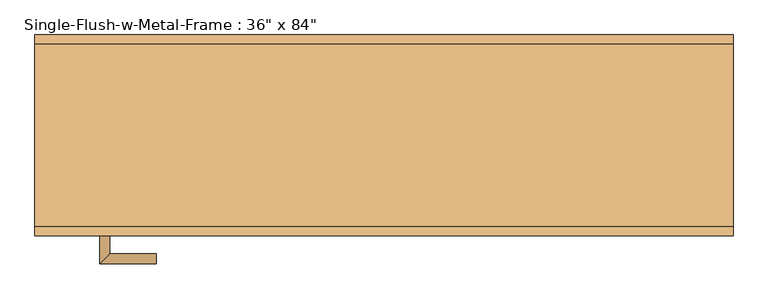
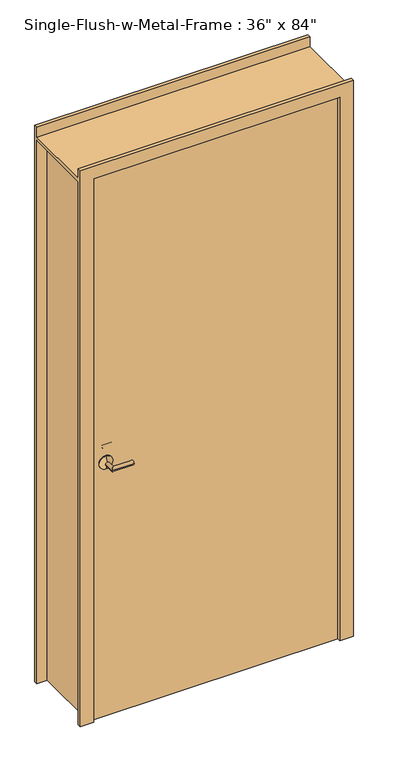
"""IFC4 building model written with IfcOpenShell, lengths in millimetres: door geometry."""

from ifc_helpers import new_model, si_unit, point, frame, origin, origin_with_axes, place, context, project, spatial, polyline, circle_curve, ellipse_curve, trimmed, outline, extrude, faceted_brep, source, transform, mapped, element, save
from ifc_brep_helpers import plane_surface, cylinder_surface, revolved_surface, advanced_brep


def door_4c242799(model_context):
    return source(origin(), model_context, "Body", "SolidModel", [
        advanced_brep(
        [(-406.4, -79.375, 971.55), (-406.4, -79.375, 1022.35), (-406.4, -70.8863821, 1004.45), (-413.9, -70.8863821, 996.95), (-406.4, -70.8863821, 989.45), (-398.9, -70.8863821, 996.95), (-406.4, -82.55, 971.55), (-406.4, -82.55, 1022.35), (-406.4, -82.55, 996.95), (-413.9, -28.95, 996.95), (-398.9, -43.95, 996.95), (-331.4, -28.95, 996.95), (-331.4, -43.95, 996.95)],
        [
            (0, 1, circle_curve(frame((-406.4, -79.375, 996.95), z_axis=(0.0, 1.0, 0.0), x_axis=(0.0, 0.0, 1.0)), 25.4)),
            (1, 2, circle_curve(frame((-406.4, -42.7707225, 1028.7458887), z_axis=(1.0, 0.0, 0.0), x_axis=(0.0, 0.0, -1.0)), 37.1588553)),
            (2, 3, circle_curve(frame((-406.4, -70.8863821, 996.95), z_axis=(0.0, -1.0, 0.0), x_axis=(0.0, 0.0, 1.0)), 7.5)),
            (3, 4, circle_curve(frame((-406.4, -70.8863821, 996.95), z_axis=(0.0, -1.0, 0.0), x_axis=(0.0, 0.0, 1.0)), 7.5)),
            (4, 0, circle_curve(frame((-406.4, -42.7707225, 965.1541113), z_axis=(1.0, 0.0, 0.0), x_axis=(0.0, 0.0, 1.0)), 37.1588553)),
            (1, 0, circle_curve(frame((-406.4, -79.375, 996.95), z_axis=(0.0, 1.0, 0.0), x_axis=(0.0, 0.0, 1.0)), 25.4)),
            (4, 5, circle_curve(frame((-406.4, -70.8863821, 996.95), z_axis=(0.0, -1.0, 0.0), x_axis=(0.0, 0.0, 1.0)), 7.5)),
            (5, 2, circle_curve(frame((-406.4, -70.8863821, 996.95), z_axis=(0.0, -1.0, 0.0), x_axis=(0.0, 0.0, 1.0)), 7.5)),
            (0, 6),
            (6, 7, circle_curve(frame((-406.4, -82.55, 996.95), z_axis=(0.0, 1.0, 0.0), x_axis=(0.0, 0.0, 1.0)), 25.4)),
            (7, 1),
            (7, 6, circle_curve(frame((-406.4, -82.55, 996.95), z_axis=(0.0, 1.0, 0.0), x_axis=(0.0, 0.0, 1.0)), 25.4)),
            (6, 8),
            (8, 7),
            (9, 10, ellipse_curve(frame((-406.4, -36.45, 996.95), z_axis=(-0.7071067811864695, -0.7071067811866254, 0.0), x_axis=(0.7071067811866254, -0.7071067811864696, 0.0)), 10.6066017, 7.5)),
            (10, 5),
            (3, 9),
            (10, 9, ellipse_curve(frame((-406.4, -36.45, 996.95), z_axis=(-0.7071067811864695, -0.7071067811866254, 0.0), x_axis=(0.7071067811866254, -0.7071067811864696, 0.0)), 10.6066017, 7.5)),
            (11, 12, circle_curve(frame((-331.4, -36.45, 996.95), z_axis=(1.0, 0.0, 0.0), x_axis=(0.0, -1.0, 0.0)), 7.5)),
            (12, 11, circle_curve(frame((-331.4, -36.45, 996.95), z_axis=(1.0, 0.0, 0.0), x_axis=(0.0, -1.0, 0.0)), 7.5)),
            (9, 11),
            (12, 10),
        ],
        [
            revolved_surface(trimmed(ellipse_curve(frame((-406.4, -42.7707225, 1028.7458887), z_axis=(-1.0, 0.0, 0.0), x_axis=(0.0, 0.0, -1.0)), 37.1588553, 37.1588553), [point((-406.4, -69.85, 1003.3))], [point((-406.4, -79.375, 1022.35))], True, "CARTESIAN"), (-406.4, -69.85, 996.95), (0.0, -1.0, 0.0)),
            cylinder_surface(frame((-406.4, -69.85, 996.95), z_axis=(0.0, -1.0, 0.0), x_axis=(0.0, 0.0, 1.0)), 25.4),
            plane_surface(frame((-406.4, -82.55, 996.95), z_axis=(0.0, -1.0, 0.0), x_axis=(0.0, 0.0, 1.0))),
            cylinder_surface(frame((-406.4, -74.55, 996.95), z_axis=(0.0, -1.0, 0.0), x_axis=(1.0, 0.0, 0.0)), 7.5),
            plane_surface(frame((-331.4, -36.45, 996.95), z_axis=(1.0, 0.0, 0.0), x_axis=(0.0, 0.0, 1.0))),
            cylinder_surface(frame((-406.4, -36.45, 996.95), z_axis=(-1.0, 0.0, 0.0), x_axis=(0.0, -1.0, 0.0)), 7.5),
        ],
        [
            (0, [[1, 2, 3, 4, 5]]),
            (0, [[6, -5, 7, 8, -2]]),
            (1, [[-1, 9, 10, 11]]),
            (1, [[-6, -11, 12, -9]]),
            (2, [[-10, 13, 14]]),
            (2, [[-12, -14, -13]]),
            (3, [[15, 16, -7, -4, 17]]),
            (3, [[18, -17, -3, -8, -16]]),
            (4, [[19, 20]]),
            (5, [[-15, 21, -20, 22]]),
            (5, [[-18, -22, -19, -21]]),
        ],
    ),
        advanced_brep(
        [(-406.4, -136.525, 971.55), (-406.4, -145.0136179, 989.45), (-413.9, -145.0136179, 996.95), (-406.4, -145.0136179, 1004.45), (-406.4, -136.525, 1022.35), (-398.9, -145.0136179, 996.95), (-406.4, -133.35, 1022.35), (-406.4, -133.35, 971.55), (-406.4, -133.35, 996.95), (-413.9, -186.95, 996.95), (-398.9, -171.95, 996.95), (-331.4, -186.95, 996.95), (-331.4, -171.95, 996.95)],
        [
            (0, 1, circle_curve(frame((-406.4, -173.1292775, 965.1541113), z_axis=(1.0, 0.0, 0.0), x_axis=(0.0, 0.0, 1.0)), 37.1588553)),
            (1, 2, circle_curve(frame((-406.4, -145.0136179, 996.95), z_axis=(0.0, 1.0, 0.0), x_axis=(0.0, 0.0, 1.0)), 7.5)),
            (2, 3, circle_curve(frame((-406.4, -145.0136179, 996.95), z_axis=(0.0, 1.0, 0.0), x_axis=(0.0, 0.0, 1.0)), 7.5)),
            (3, 4, circle_curve(frame((-406.4, -173.1292775, 1028.7458887), z_axis=(1.0, 0.0, 0.0), x_axis=(0.0, 0.0, -1.0)), 37.1588553)),
            (4, 0, circle_curve(frame((-406.4, -136.525, 996.95), z_axis=(0.0, -1.0, 0.0), x_axis=(0.0, 0.0, 1.0)), 25.4)),
            (3, 5, circle_curve(frame((-406.4, -145.0136179, 996.95), z_axis=(0.0, 1.0, 0.0), x_axis=(0.0, 0.0, 1.0)), 7.5)),
            (5, 1, circle_curve(frame((-406.4, -145.0136179, 996.95), z_axis=(0.0, 1.0, 0.0), x_axis=(0.0, 0.0, 1.0)), 7.5)),
            (0, 4, circle_curve(frame((-406.4, -136.525, 996.95), z_axis=(0.0, -1.0, 0.0), x_axis=(0.0, 0.0, 1.0)), 25.4)),
            (4, 6),
            (6, 7, circle_curve(frame((-406.4, -133.35, 996.95), z_axis=(0.0, -1.0, 0.0), x_axis=(0.0, 0.0, 1.0)), 25.4)),
            (7, 0),
            (7, 6, circle_curve(frame((-406.4, -133.35, 996.95), z_axis=(0.0, -1.0, 0.0), x_axis=(0.0, 0.0, 1.0)), 25.4)),
            (6, 8),
            (8, 7),
            (9, 2),
            (5, 10),
            (10, 9, ellipse_curve(frame((-406.4, -179.45, 996.95), z_axis=(-0.7071067811864695, 0.7071067811866254, 0.0), x_axis=(0.7071067811866254, 0.7071067811864696, 0.0)), 10.6066017, 7.5)),
            (9, 10, ellipse_curve(frame((-406.4, -179.45, 996.95), z_axis=(-0.7071067811864695, 0.7071067811866254, 0.0), x_axis=(0.7071067811866254, 0.7071067811864696, 0.0)), 10.6066017, 7.5)),
            (11, 12, circle_curve(frame((-331.4, -179.45, 996.95), z_axis=(1.0, 0.0, 0.0), x_axis=(0.0, 1.0, 0.0)), 7.5)),
            (12, 11, circle_curve(frame((-331.4, -179.45, 996.95), z_axis=(1.0, 0.0, 0.0), x_axis=(0.0, 1.0, 0.0)), 7.5)),
            (10, 12),
            (11, 9),
        ],
        [
            revolved_surface(trimmed(ellipse_curve(frame((-406.4, -173.1292775, 1028.7458887), z_axis=(1.0, 0.0, 0.0), x_axis=(0.0, 0.0, -1.0)), 37.1588553, 37.1588553), [point((-406.4, -146.05, 1003.3))], [point((-406.4, -136.525, 1022.35))], True, "CARTESIAN"), (-406.4, -146.05, 996.95), (0.0, 1.0, 0.0)),
            cylinder_surface(frame((-406.4, -146.05, 996.95), z_axis=(0.0, 1.0, 0.0), x_axis=(0.0, 0.0, 1.0)), 25.4),
            plane_surface(frame((-406.4, -133.35, 996.95), z_axis=(0.0, 1.0, 0.0), x_axis=(0.0, 0.0, 1.0))),
            cylinder_surface(frame((-406.4, -141.35, 996.95), z_axis=(0.0, 1.0, 0.0), x_axis=(1.0, 0.0, 0.0)), 7.5),
            plane_surface(frame((-331.4, -179.45, 996.95), z_axis=(1.0, 0.0, 0.0), x_axis=(0.0, 0.0, 1.0))),
            cylinder_surface(frame((-406.4, -179.45, 996.95), z_axis=(-1.0, 0.0, 0.0), x_axis=(0.0, 1.0, 0.0)), 7.5),
        ],
        [
            (0, [[1, 2, 3, 4, 5]]),
            (0, [[-4, 6, 7, -1, 8]]),
            (1, [[9, 10, 11, -5]]),
            (1, [[-11, 12, -9, -8]]),
            (2, [[13, 14, -10]]),
            (2, [[-14, -13, -12]]),
            (3, [[15, -2, -7, 16, 17]]),
            (3, [[-16, -6, -3, -15, 18]]),
            (4, [[19, 20]]),
            (5, [[21, -19, 22, -17]]),
            (5, [[-22, -20, -21, -18]]),
        ],
    ),
        extrude(outline(polyline([(457.2, -82.55), (457.2, -133.35), (-457.2, -133.35), (-457.2, -82.55), (457.2, -82.55)])), origin_with_axes(), (0.0, 0.0, 1.0), 2133.6),
        faceted_brep([(-469.9, -133.35, 0.0), (-469.9, 133.35, 0.0), (-508.0, 133.35, 0.0), (-508.0, 146.05, 0.0), (-457.2, 146.05, 0.0), (-457.2, -146.05, 0.0), (-508.0, -146.05, 0.0), (-508.0, -133.35, 0.0), (-508.0, -133.35, 2133.6), (-469.9, -133.35, 2133.6), (-508.0, -146.05, 2184.4), (-508.0, -133.35, 2184.4), (-508.0, -133.35, 2146.3), (-508.0, 133.35, 2146.3), (-508.0, 133.35, 2184.4), (-508.0, 146.05, 2184.4), (-508.0, 133.35, 2133.6), (-457.2, -146.05, 2133.6), (457.2, -146.05, 2133.6), (457.2, -146.05, 0.0), (508.0, -146.05, 0.0), (508.0, -146.05, 2184.4), (-457.2, 146.05, 2133.6), (508.0, 146.05, 2184.4), (508.0, 146.05, 0.0), (457.2, 146.05, 0.0), (457.2, 146.05, 2133.6), (-469.9, 133.35, 2133.6), (469.9, -133.35, 0.0), (508.0, -133.35, 0.0), (508.0, 133.35, 0.0), (469.9, 133.35, 0.0), (508.0, 133.35, 2146.3), (508.0, -133.35, 2146.3), (508.0, -133.35, 2184.4), (508.0, -133.35, 2133.6), (508.0, 133.35, 2133.6), (508.0, 133.35, 2184.4), (469.9, 133.35, 2133.6), (469.9, -133.35, 2133.6)], [[[0, 1, 2, 3, 4, 5, 6, 7]], [[7, 8, 9, 0]], [[6, 10, 11, 12, 13, 14, 15, 3, 2, 16, 8, 7]], [[5, 17, 18, 19, 20, 21, 10, 6]], [[4, 22, 17, 5]], [[3, 15, 23, 24, 25, 26, 22, 4]], [[1, 27, 16, 2]], [[0, 9, 27, 1]], [[19, 18, 26, 25]], [[28, 29, 20, 19, 25, 24, 30, 31]], [[32, 33, 34, 21, 20, 29, 35, 36, 30, 24, 23, 37]], [[30, 36, 38, 31]], [[28, 39, 35, 29]], [[31, 38, 39, 28]], [[37, 14, 13, 32]], [[23, 15, 14, 37]], [[16, 27, 9, 8]], [[22, 26, 18, 17]], [[35, 39, 38, 36]], [[34, 11, 10, 21]], [[33, 12, 11, 34]], [[32, 13, 12, 33]]]),
    ])


if __name__ == "__main__":
    model = new_model("IFC4")
    model_context = context("Model", 3, world=origin())
    ifc_project = project(units=[si_unit("LENGTHUNIT", "METRE", prefix="MILLI")], contexts=[model_context])
    site = spatial("IfcSite", under=ifc_project)
    building = spatial("IfcBuilding", under=site)
    placement = place(None, origin())
    door_shape = door_4c242799(model_context)
    element("IfcDoor", 1, ObjectType="Single-Flush-w-Metal-Frame : 36\" x 84\"", at=placement, inside=building, context=model_context, shape_type="MappedRepresentation", body=[
        mapped(door_shape, transform((0.0, 0.0, 0.0), x_axis=(1.0, 0.0, 0.0), y_axis=(0.0, 1.0, 0.0), z_axis=(0.0, 0.0, 1.0))),
    ])
    save(model, "model.ifc")

# Revit data of these elements
# Type "Single-Flush-w-Metal-Frame : 36\" x 84\""
#   Type Mark = "16"
#   Construction Type Id = "MDOOR"
#   Assembly Code = "C1020"
#   Analytic Construction = "Metal"
#   Thickness = 0' - 2"
#   Thermal Resistance (R) = 1.5338 (h·ft²·°F)/BTU
#   Half Width Neg = -1' - 8"
#   Half Width = 1' - 8"
#   Frame Width = 0' - 2"
#   Frame Thickness = 0' - 0 1/2"
#   Frame Head Height = 0' - 2"
#   Heat Transfer Coefficient (U) = 0.651978 BTU/(h·ft²·°F)
#   Height = 7' - 0"
#   Width = 3' - 0"
#   Define Thermal Properties by = 1
#   Define Thermal Properties by = 1
#   Door Material = Door - Panel
#   Frame Material = Door - Frame
#   Visual Light Transmittance = 0
#   Solar Heat Gain Coefficient = 0
#   Function = (empty or 0)
#   Wall Closure = (empty or 0)
# Element 1 (IfcDoor, "Single-Flush-w-Metal-Frame : 36\" x 84\"")
#   Materials on its faces: "Metal - Aluminium", "Door - Frame", "Door - Panel"
# Materials
#   "Door - Panel": class "Wood", colour RGB 210 159 95, transparency 0
#   "Door - Frame": class "Miscellaneous", colour RGB 118 70 51, transparency 0
#   "Metal - Aluminium": class "Unassigned", colour RGB 247 247 247, transparency 0
